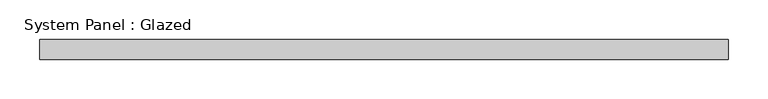
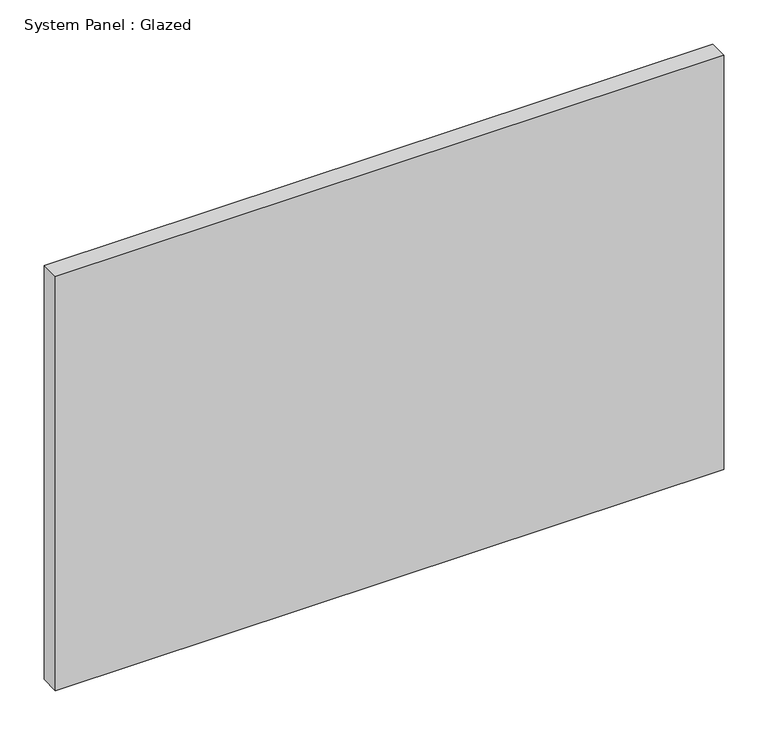
"""IFC4 building model written with IfcOpenShell, lengths in millimetres: plate geometry, System Panel : Glazed."""

import ifcopenshell
import ifcopenshell.guid

model = None  # the IFC model being written
_history = None  # IfcOwnerHistory: only IFC2X3 demands one
_inside = {}  # id of a spatial element -> (the spatial element, [elements in it])
_under = {}  # id of a project, library or spatial element -> (it, [spatial elements below it])
_declared = {}  # id of a project -> (the project, [libraries it declares])
_typed = {}  # id of a type object -> (the type object, [elements of that type])
_made_of = {}  # id of a material, layer set ... -> (it, [elements and type objects made of it])


def new_model(schema):
    """Start an empty IFC model of exactly this schema.

    Asked for "IFC4X3", IfcOpenShell would pick the latest addendum, in which some entities
    have other attributes; the version numbers below select the first issue.
    IFC2X3 requires an IfcOwnerHistory on every rooted entity: one is made here for all.
    """
    global model, _history
    if schema == "IFC4X3":
        model = ifcopenshell.file(schema_version=(4, 3, 0, 0))
    else:
        model = ifcopenshell.file(schema=schema)
    _inside.clear()
    _under.clear()
    _declared.clear()
    _typed.clear()
    _made_of.clear()
    _history = None
    if model.schema == "IFC2X3":
        org = make("IfcOrganization", Name="unknown")
        user = make(
            "IfcPersonAndOrganization",
            ThePerson=make("IfcPerson", FamilyName="unknown"),
            TheOrganization=org,
        )
        app = make(
            "IfcApplication",
            ApplicationDeveloper=org,
            Version="unknown",
            ApplicationFullName="unknown",
            ApplicationIdentifier="unknown",
        )
        _history = make(
            "IfcOwnerHistory",
            OwningUser=user,
            OwningApplication=app,
            ChangeAction="ADDED",
            CreationDate=0,
        )
    return model


def make(cls, **values):
    """One entity of the class cls with the attributes given. An attribute that is None is left unset."""
    return model.create_entity(
        cls, **{name: value for name, value in values.items() if value is not None}
    )


def rooted(cls, **values):
    """An entity with a GlobalId (a new one), such as an element, a storey or a relation."""
    return make(cls, GlobalId=ifcopenshell.guid.new(), OwnerHistory=_history, **values)


def si_unit(unit_type, name, prefix=None):
    """IfcSIUnit, for example si_unit("LENGTHUNIT", "METRE", prefix="MILLI")."""
    return make("IfcSIUnit", UnitType=unit_type, Prefix=prefix, Name=name)


def assignment(units):
    """IfcUnitAssignment: the units of a project."""
    return None if units is None else make("IfcUnitAssignment", Units=units)


def point(xyz):
    """IfcCartesianPoint."""
    return None if xyz is None else make("IfcCartesianPoint", Coordinates=xyz)


def direction(xyz):
    """IfcDirection."""
    return None if xyz is None else make("IfcDirection", DirectionRatios=xyz)


def frame(location, z_axis=None, x_axis=None):
    """IfcAxis2Placement3D, a coordinate frame: its origin and axes. An axis left out is left unset."""
    return make(
        "IfcAxis2Placement3D",
        Location=point(location),
        Axis=direction(z_axis),
        RefDirection=direction(x_axis),
    )


def origin():
    """The frame at (0, 0, 0) with its axes left unset."""
    return frame((0.0, 0.0, 0.0))


def origin_with_axes():
    """The frame at (0, 0, 0) with the z axis (0, 0, 1) and the x axis (1, 0, 0) written out."""
    return frame((0.0, 0.0, 0.0), z_axis=(0.0, 0.0, 1.0), x_axis=(1.0, 0.0, 0.0))


def place(relative_to, where):
    """IfcLocalPlacement: puts the frame where relative to a parent placement (None: the world)."""
    return make(
        "IfcLocalPlacement", PlacementRelTo=relative_to, RelativePlacement=where
    )


def context(
    kind, dimensions, precision=None, world=None, true_north=None, identifier=None
):
    """IfcGeometricRepresentationContext, for example the 3D "Model" context."""
    return make(
        "IfcGeometricRepresentationContext",
        ContextIdentifier=identifier,
        ContextType=kind,
        CoordinateSpaceDimension=dimensions,
        Precision=precision,
        WorldCoordinateSystem=world,
        TrueNorth=true_north,
    )


def project(units=None, contexts=None):
    """IfcProject with its units and contexts."""
    return rooted(
        "IfcProject",
        Name="project",
        RepresentationContexts=contexts,
        UnitsInContext=assignment(units),
    )


def spatial(cls, under=None, at=None, **own):
    """A site, building, storey or space (cls), placed at a placement, below another one or the project."""
    s = rooted(cls, ObjectPlacement=at, **own)
    if under is not None:
        _under.setdefault(under.id(), (under, []))[1].append(s)
    return s


def polyline(points):
    """IfcPolyline through the points."""
    return make("IfcPolyline", Points=[point(p) for p in points])


def outline(outer, holes=None, kind="AREA"):
    """IfcArbitraryClosedProfileDef: a profile drawn as a closed curve; with holes, ...WithVoids."""
    if holes is None:
        return make("IfcArbitraryClosedProfileDef", ProfileType=kind, OuterCurve=outer)
    return make(
        "IfcArbitraryProfileDefWithVoids",
        ProfileType=kind,
        OuterCurve=outer,
        InnerCurves=holes,
    )


def extrude(swept, where, along, depth):
    """IfcExtrudedAreaSolid: the profile swept, set in the frame where, extruded along a direction by depth."""
    return make(
        "IfcExtrudedAreaSolid",
        SweptArea=swept,
        Position=where,
        ExtrudedDirection=direction(along),
        Depth=depth,
    )


def shape(context_of_items, identifier, shape_type, items):
    """IfcShapeRepresentation: the items that make up one representation, for example the "Body"."""
    return make(
        "IfcShapeRepresentation",
        ContextOfItems=context_of_items,
        RepresentationIdentifier=identifier,
        RepresentationType=shape_type,
        Items=items,
    )


def source(mapping_origin, context_of_items, identifier, shape_type, items):
    """IfcRepresentationMap: a shape defined once, which mapped items show again and again."""
    return make(
        "IfcRepresentationMap",
        MappingOrigin=mapping_origin,
        MappedRepresentation=shape(context_of_items, identifier, shape_type, items),
    )


def transform(
    local_origin,
    x_axis=None,
    y_axis=None,
    z_axis=None,
    scale=None,
    scale2=None,
    scale3=None,
    uniform=True,
):
    """IfcCartesianTransformationOperator3D, or its non-uniform kind. x_axis, y_axis, z_axis: its Axis1, 2, 3."""
    if uniform:
        return make(
            "IfcCartesianTransformationOperator3D",
            Axis1=direction(x_axis),
            Axis2=direction(y_axis),
            LocalOrigin=point(local_origin),
            Scale=scale,
            Axis3=direction(z_axis),
        )
    return make(
        "IfcCartesianTransformationOperator3DnonUniform",
        Axis1=direction(x_axis),
        Axis2=direction(y_axis),
        LocalOrigin=point(local_origin),
        Scale=scale,
        Axis3=direction(z_axis),
        Scale2=scale2,
        Scale3=scale3,
    )


def mapped(mapping_source, mapping_target):
    """IfcMappedItem: shows the shape of a source again, moved by a transform."""
    return make(
        "IfcMappedItem", MappingSource=mapping_source, MappingTarget=mapping_target
    )


def made_of(thing, what):
    """Note that an element or type object is made of a material, layer set ...; save() writes the relation."""
    if what is not None:
        _made_of.setdefault(what.id(), (what, []))[1].append(thing)
    return thing


def element(
    cls,
    number,
    at=None,
    inside=None,
    cuts=None,
    type_object=None,
    material=None,
    context=None,
    identifier="Body",
    shape_type=None,
    held_by="IfcProductDefinitionShape",
    body=None,
    shapes=None,
    **own,
):
    """One element of the class cls, such as IfcWall. Its Tag is "e" and its number.

    at: its placement. inside: the storey or other place that contains it. cuts: it is an
    opening in that element (IfcRelVoidsElement). A single representation is given by context,
    identifier, shape_type and body (its items); several are given by shapes. held_by: the class
    of the entity that holds the representations. save() writes the other relations.
    """
    e = rooted(cls, Tag="e%d" % number, ObjectPlacement=at, **own)
    if body is not None:
        shapes = [shape(context, identifier, shape_type, body)]
    if shapes is not None:
        e.Representation = make(held_by, Representations=shapes)
    if inside is not None:
        _inside.setdefault(inside.id(), (inside, []))[1].append(e)
    if cuts is not None:
        rooted(
            "IfcRelVoidsElement", RelatingBuildingElement=cuts, RelatedOpeningElement=e
        )
    if type_object is not None:
        _typed.setdefault(type_object.id(), (type_object, []))[1].append(e)
    return made_of(e, material)


def aggregate(whole, parts):
    """IfcRelAggregates: a whole, such as a stair, and the parts it consists of."""
    return rooted("IfcRelAggregates", RelatingObject=whole, RelatedObjects=parts)


def save(model, path):
    """Write the relations noted so far, then the file.

    IfcRelAggregates (storeys below a building ...), IfcRelContainedInSpatialStructure (elements
    in a storey), IfcRelDefinesByType, IfcRelAssociatesMaterial and IfcRelDeclares: one each for
    every whole, place, type object, material and project.
    """
    for whole, parts in _under.values():
        aggregate(whole, parts)
    for where, things in _inside.values():
        rooted(
            "IfcRelContainedInSpatialStructure",
            RelatedElements=things,
            RelatingStructure=where,
        )
    for kind, things in _typed.values():
        rooted("IfcRelDefinesByType", RelatedObjects=things, RelatingType=kind)
    for what, things in _made_of.values():
        rooted("IfcRelAssociatesMaterial", RelatedObjects=things, RelatingMaterial=what)
    for by, libraries in _declared.values():
        rooted("IfcRelDeclares", RelatingContext=by, RelatedDefinitions=libraries)
    model.write(path)


def system_panel_glazed_1c5266c5(model_context):
    return source(origin(), model_context, "Body", "SweptSolid", [
        extrude(outline(polyline([(435.9649128, 19.05), (-435.9649128, 19.05), (-435.9649128, 44.45), (435.9649128, 44.45), (435.9649128, 19.05)])), origin_with_axes(), (0.0, 0.0, 1.0), 571.5),
    ])


if __name__ == "__main__":
    model = new_model("IFC4")
    model_context = context("Model", 3, world=origin())
    ifc_project = project(units=[si_unit("LENGTHUNIT", "METRE", prefix="MILLI")], contexts=[model_context])
    site = spatial("IfcSite", under=ifc_project)
    building = spatial("IfcBuilding", under=site)
    placement = place(None, origin())
    system_panel_glazed_shape = system_panel_glazed_1c5266c5(model_context)
    element("IfcPlate", 1, ObjectType="System Panel : Glazed", at=placement, inside=building, context=model_context, shape_type="MappedRepresentation", body=[
        mapped(system_panel_glazed_shape, transform((0.0, 0.0, 0.0), x_axis=(1.0, 0.0, 0.0), y_axis=(0.0, 1.0, 0.0), z_axis=(0.0, 0.0, 1.0))),
    ])
    save(model, "model.ifc")

# Revit data of these elements
# Type "System Panel : Glazed"
#   Construction Type Id = "GSP4R"
#   Analytic Construction = "1/8 in Pilkington single glazing"
#   Visual Light Transmittance = 0.9
#   Solar Heat Gain Coefficient = 0.86
#   Heat Transfer Coefficient (U) = 1.18115 BTU/(h·ft²·°F)
#   Define Thermal Properties by = 1
# Element 1 (IfcPlate, "System Panel : Glazed")
#   Materials on its faces: "Glass"
# Materials
#   "Glass": class "Glass", colour RGB 0 128 192, transparency 0.75, Description = "Soda Lime Glass", Cost = 0
